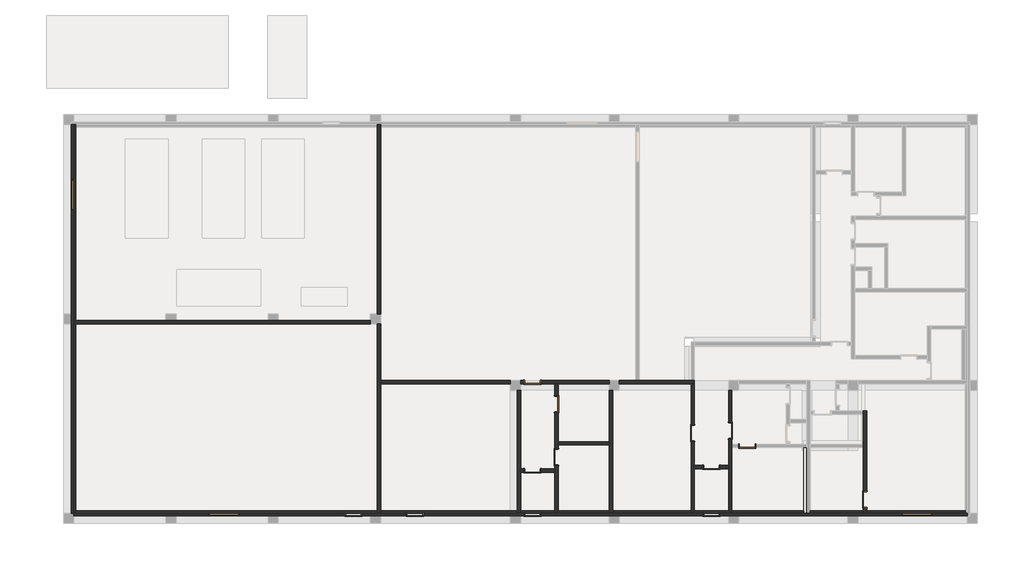
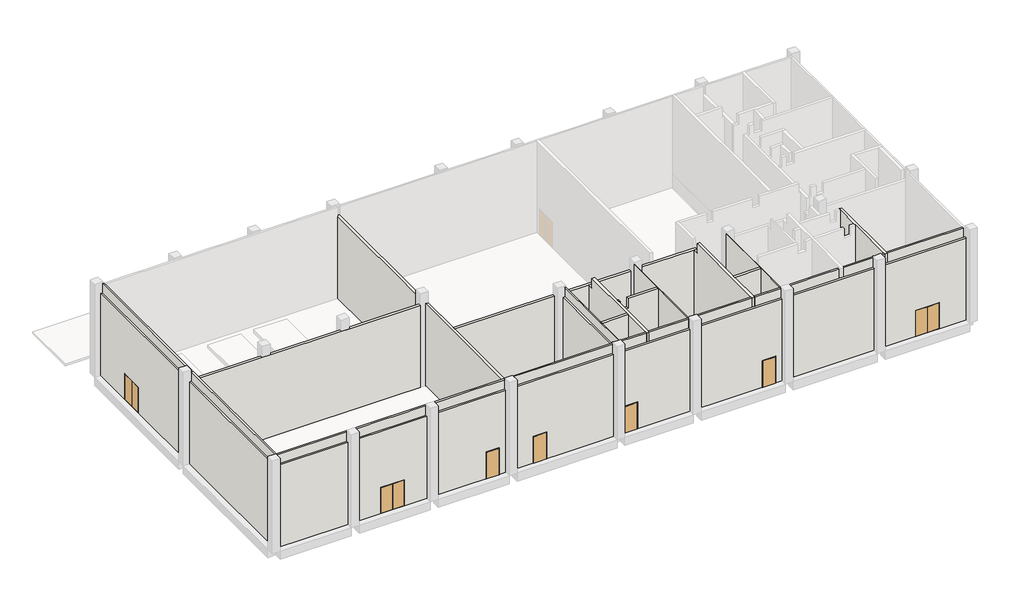
# One storey, part 1 of 4: 31 walls, 16 doors.
"""IFC4 building model written with IfcOpenShell, lengths in millimetres."""

import ifcopenshell
import ifcopenshell.guid

model = None  # the IFC model being written
_history = None  # IfcOwnerHistory: only IFC2X3 demands one
_inside = {}  # id of a spatial element -> (the spatial element, [elements in it])
_under = {}  # id of a project, library or spatial element -> (it, [spatial elements below it])
_declared = {}  # id of a project -> (the project, [libraries it declares])
_typed = {}  # id of a type object -> (the type object, [elements of that type])
_made_of = {}  # id of a material, layer set ... -> (it, [elements and type objects made of it])


def new_model(schema):
    """Start an empty IFC model of exactly this schema.

    Asked for "IFC4X3", IfcOpenShell would pick the latest addendum, in which some entities
    have other attributes; the version numbers below select the first issue.
    IFC2X3 requires an IfcOwnerHistory on every rooted entity: one is made here for all.
    """
    global model, _history
    if schema == "IFC4X3":
        model = ifcopenshell.file(schema_version=(4, 3, 0, 0))
    else:
        model = ifcopenshell.file(schema=schema)
    _inside.clear()
    _under.clear()
    _declared.clear()
    _typed.clear()
    _made_of.clear()
    _history = None
    if model.schema == "IFC2X3":
        org = make("IfcOrganization", Name="unknown")
        user = make(
            "IfcPersonAndOrganization",
            ThePerson=make("IfcPerson", FamilyName="unknown"),
            TheOrganization=org,
        )
        app = make(
            "IfcApplication",
            ApplicationDeveloper=org,
            Version="unknown",
            ApplicationFullName="unknown",
            ApplicationIdentifier="unknown",
        )
        _history = make(
            "IfcOwnerHistory",
            OwningUser=user,
            OwningApplication=app,
            ChangeAction="ADDED",
            CreationDate=0,
        )
    return model


def make(cls, **values):
    """One entity of the class cls with the attributes given. An attribute that is None is left unset."""
    return model.create_entity(
        cls, **{name: value for name, value in values.items() if value is not None}
    )


def rooted(cls, **values):
    """An entity with a GlobalId (a new one), such as an element, a storey or a relation."""
    return make(cls, GlobalId=ifcopenshell.guid.new(), OwnerHistory=_history, **values)


def si_unit(unit_type, name, prefix=None):
    """IfcSIUnit, for example si_unit("LENGTHUNIT", "METRE", prefix="MILLI")."""
    return make("IfcSIUnit", UnitType=unit_type, Prefix=prefix, Name=name)


def assignment(units):
    """IfcUnitAssignment: the units of a project."""
    return None if units is None else make("IfcUnitAssignment", Units=units)


def point(xyz):
    """IfcCartesianPoint."""
    return None if xyz is None else make("IfcCartesianPoint", Coordinates=xyz)


def direction(xyz):
    """IfcDirection."""
    return None if xyz is None else make("IfcDirection", DirectionRatios=xyz)


def frame(location, z_axis=None, x_axis=None):
    """IfcAxis2Placement3D, a coordinate frame: its origin and axes. An axis left out is left unset."""
    return make(
        "IfcAxis2Placement3D",
        Location=point(location),
        Axis=direction(z_axis),
        RefDirection=direction(x_axis),
    )


def origin():
    """The frame at (0, 0, 0) with its axes left unset."""
    return frame((0.0, 0.0, 0.0))


def origin_with_axes():
    """The frame at (0, 0, 0) with the z axis (0, 0, 1) and the x axis (1, 0, 0) written out."""
    return frame((0.0, 0.0, 0.0), z_axis=(0.0, 0.0, 1.0), x_axis=(1.0, 0.0, 0.0))


def place(relative_to, where):
    """IfcLocalPlacement: puts the frame where relative to a parent placement (None: the world)."""
    return make(
        "IfcLocalPlacement", PlacementRelTo=relative_to, RelativePlacement=where
    )


def context(
    kind, dimensions, precision=None, world=None, true_north=None, identifier=None
):
    """IfcGeometricRepresentationContext, for example the 3D "Model" context."""
    return make(
        "IfcGeometricRepresentationContext",
        ContextIdentifier=identifier,
        ContextType=kind,
        CoordinateSpaceDimension=dimensions,
        Precision=precision,
        WorldCoordinateSystem=world,
        TrueNorth=true_north,
    )


def project(units=None, contexts=None):
    """IfcProject with its units and contexts."""
    return rooted(
        "IfcProject",
        Name="project",
        RepresentationContexts=contexts,
        UnitsInContext=assignment(units),
    )


def spatial(cls, under=None, at=None, **own):
    """A site, building, storey or space (cls), placed at a placement, below another one or the project."""
    s = rooted(cls, ObjectPlacement=at, **own)
    if under is not None:
        _under.setdefault(under.id(), (under, []))[1].append(s)
    return s


def polyline(points):
    """IfcPolyline through the points."""
    return make("IfcPolyline", Points=[point(p) for p in points])


def outline(outer, holes=None, kind="AREA"):
    """IfcArbitraryClosedProfileDef: a profile drawn as a closed curve; with holes, ...WithVoids."""
    if holes is None:
        return make("IfcArbitraryClosedProfileDef", ProfileType=kind, OuterCurve=outer)
    return make(
        "IfcArbitraryProfileDefWithVoids",
        ProfileType=kind,
        OuterCurve=outer,
        InnerCurves=holes,
    )


def extrude(swept, where, along, depth):
    """IfcExtrudedAreaSolid: the profile swept, set in the frame where, extruded along a direction by depth."""
    return make(
        "IfcExtrudedAreaSolid",
        SweptArea=swept,
        Position=where,
        ExtrudedDirection=direction(along),
        Depth=depth,
    )


def faces_of(points, faces, orient=None, outer=None):
    """IfcFace entities. A face is a list of loops; a loop is a list of indices into points, from 0.

    orient and outer hold one flag for each loop. By default every Orientation is true, the
    first loop of a face is its IfcFaceOuterBound and the others are IfcFaceBound.
    """
    made = []
    for i, loops in enumerate(faces):
        bounds = []
        for j, loop in enumerate(loops):
            is_outer = j == 0 if outer is None else outer[i][j]
            bounds.append(
                make(
                    "IfcFaceOuterBound" if is_outer else "IfcFaceBound",
                    Bound=make("IfcPolyLoop", Polygon=[points[k] for k in loop]),
                    Orientation=True if orient is None else orient[i][j],
                )
            )
        made.append(make("IfcFace", Bounds=bounds))
    return made


def faceted_brep(points, faces, orient=None, outer=None, voids=None):
    """IfcFacetedBrep: a solid bounded by flat faces; with voids (closed shells), ...WithVoids."""
    shared = [point(p) for p in points]
    hull = make("IfcClosedShell", CfsFaces=faces_of(shared, faces, orient, outer))
    if voids is None:
        return make("IfcFacetedBrep", Outer=hull)
    return make(
        "IfcFacetedBrepWithVoids",
        Outer=hull,
        Voids=[
            make(cls, CfsFaces=faces_of(shared, fs, o, b)) for cls, fs, o, b in voids
        ],
    )


def shape(context_of_items, identifier, shape_type, items):
    """IfcShapeRepresentation: the items that make up one representation, for example the "Body"."""
    return make(
        "IfcShapeRepresentation",
        ContextOfItems=context_of_items,
        RepresentationIdentifier=identifier,
        RepresentationType=shape_type,
        Items=items,
    )


def source(mapping_origin, context_of_items, identifier, shape_type, items):
    """IfcRepresentationMap: a shape defined once, which mapped items show again and again."""
    return make(
        "IfcRepresentationMap",
        MappingOrigin=mapping_origin,
        MappedRepresentation=shape(context_of_items, identifier, shape_type, items),
    )


def transform(
    local_origin,
    x_axis=None,
    y_axis=None,
    z_axis=None,
    scale=None,
    scale2=None,
    scale3=None,
    uniform=True,
):
    """IfcCartesianTransformationOperator3D, or its non-uniform kind. x_axis, y_axis, z_axis: its Axis1, 2, 3."""
    if uniform:
        return make(
            "IfcCartesianTransformationOperator3D",
            Axis1=direction(x_axis),
            Axis2=direction(y_axis),
            LocalOrigin=point(local_origin),
            Scale=scale,
            Axis3=direction(z_axis),
        )
    return make(
        "IfcCartesianTransformationOperator3DnonUniform",
        Axis1=direction(x_axis),
        Axis2=direction(y_axis),
        LocalOrigin=point(local_origin),
        Scale=scale,
        Axis3=direction(z_axis),
        Scale2=scale2,
        Scale3=scale3,
    )


def mapped(mapping_source, mapping_target):
    """IfcMappedItem: shows the shape of a source again, moved by a transform."""
    return make(
        "IfcMappedItem", MappingSource=mapping_source, MappingTarget=mapping_target
    )


def made_of(thing, what):
    """Note that an element or type object is made of a material, layer set ...; save() writes the relation."""
    if what is not None:
        _made_of.setdefault(what.id(), (what, []))[1].append(thing)
    return thing


def element(
    cls,
    number,
    at=None,
    inside=None,
    cuts=None,
    type_object=None,
    material=None,
    context=None,
    identifier="Body",
    shape_type=None,
    held_by="IfcProductDefinitionShape",
    body=None,
    shapes=None,
    **own,
):
    """One element of the class cls, such as IfcWall. Its Tag is "e" and its number.

    at: its placement. inside: the storey or other place that contains it. cuts: it is an
    opening in that element (IfcRelVoidsElement). A single representation is given by context,
    identifier, shape_type and body (its items); several are given by shapes. held_by: the class
    of the entity that holds the representations. save() writes the other relations.
    """
    e = rooted(cls, Tag="e%d" % number, ObjectPlacement=at, **own)
    if body is not None:
        shapes = [shape(context, identifier, shape_type, body)]
    if shapes is not None:
        e.Representation = make(held_by, Representations=shapes)
    if inside is not None:
        _inside.setdefault(inside.id(), (inside, []))[1].append(e)
    if cuts is not None:
        rooted(
            "IfcRelVoidsElement", RelatingBuildingElement=cuts, RelatedOpeningElement=e
        )
    if type_object is not None:
        _typed.setdefault(type_object.id(), (type_object, []))[1].append(e)
    return made_of(e, material)


def aggregate(whole, parts):
    """IfcRelAggregates: a whole, such as a stair, and the parts it consists of."""
    return rooted("IfcRelAggregates", RelatingObject=whole, RelatedObjects=parts)


def save(model, path):
    """Write the relations noted so far, then the file.

    IfcRelAggregates (storeys below a building ...), IfcRelContainedInSpatialStructure (elements
    in a storey), IfcRelDefinesByType, IfcRelAssociatesMaterial and IfcRelDeclares: one each for
    every whole, place, type object, material and project.
    """
    for whole, parts in _under.values():
        aggregate(whole, parts)
    for where, things in _inside.values():
        rooted(
            "IfcRelContainedInSpatialStructure",
            RelatedElements=things,
            RelatingStructure=where,
        )
    for kind, things in _typed.values():
        rooted("IfcRelDefinesByType", RelatedObjects=things, RelatingType=kind)
    for what, things in _made_of.values():
        rooted("IfcRelAssociatesMaterial", RelatedObjects=things, RelatingMaterial=what)
    for by, libraries in _declared.values():
        rooted("IfcRelDeclares", RelatingContext=by, RelatedDefinitions=libraries)
    model.write(path)


def double_door_steel_580823b0(model_context):
    return source(origin(), model_context, "Body", "SolidModel", [
        extrude(outline(polyline([(880.0, 35.0), (0.0, 35.0), (0.0, 75.0), (880.0, 75.0), (880.0, 35.0)])), frame((0.0, 0.0, 20.0), z_axis=(0.0, 0.0, 1.0), x_axis=(1.0, 0.0, 0.0)), (0.0, 0.0, 1.0), 2060.0),
        extrude(outline(polyline([(0.0, 35.0), (-880.0, 35.0), (-880.0, 75.0), (0.0, 75.0), (0.0, 35.0)])), frame((0.0, 0.0, 20.0), z_axis=(0.0, 0.0, 1.0), x_axis=(1.0, 0.0, 0.0)), (0.0, 0.0, 1.0), 2060.0),
        faceted_brep([(900.0, -75.0, 2100.0), (900.0, 75.0, 2100.0), (-900.0, 75.0, 2100.0), (-900.0, -75.0, 2100.0), (865.0, 35.0, 2065.0), (865.0, -75.0, 2065.0), (-865.0, -75.0, 2065.0), (-865.0, 35.0, 2065.0), (880.0, 75.0, 2080.0), (880.0, 35.0, 2080.0), (-880.0, 35.0, 2080.0), (-880.0, 75.0, 2080.0), (-900.0, 75.0, 0.0), (-900.0, -75.0, 0.0), (-865.0, -75.0, 35.0), (-865.0, 35.0, 35.0), (-880.0, 35.0, 20.0), (-880.0, 75.0, 20.0), (900.0, 75.0, 0.0), (880.0, 75.0, 20.0), (900.0, -75.0, 0.0), (865.0, -75.0, 35.0), (865.0, 35.0, 35.0), (880.0, 35.0, 20.0)], [[[0, 1, 2, 3]], [[4, 5, 6, 7]], [[8, 9, 10, 11]], [[3, 2, 12, 13]], [[7, 6, 14, 15]], [[11, 10, 16, 17]], [[18, 12, 2, 1], [8, 11, 17, 19]], [[13, 12, 18, 20]], [[0, 3, 13, 20], [21, 14, 6, 5]], [[15, 14, 21, 22]], [[23, 16, 10, 9], [4, 7, 15, 22]], [[17, 16, 23, 19]], [[20, 18, 1, 0]], [[22, 21, 5, 4]], [[19, 23, 9, 8]]]),
    ])


def single_door_steel_b319cbd1(model_context):
    return source(origin(), model_context, "Body", "SolidModel", [
        extrude(outline(polyline([(480.0, -105.0), (-480.0, -105.0), (-480.0, -70.0), (480.0, -70.0), (480.0, -105.0)])), origin_with_axes(), (0.0, 0.0, 1.0), 2130.0),
        faceted_brep([(480.0, -105.0, 0.0), (480.0, -70.0, 0.0), (460.0, -70.0, 0.0), (460.0, 70.0, 0.0), (480.0, 70.0, 0.0), (480.0, 105.0, 0.0), (510.0, 105.0, 0.0), (510.0, -105.0, 0.0), (510.0, -105.0, 2160.0), (-510.0, -105.0, 2160.0), (-510.0, -105.0, 0.0), (-480.0, -105.0, 0.0), (-480.0, -105.0, 2130.0), (480.0, -105.0, 2130.0), (510.0, 105.0, 2160.0), (480.0, 105.0, 2130.0), (-480.0, 105.0, 2130.0), (-480.0, 105.0, 0.0), (-510.0, 105.0, 0.0), (-510.0, 105.0, 2160.0), (480.0, 70.0, 2130.0), (460.0, 70.0, 2110.0), (-460.0, 70.0, 2110.0), (-460.0, 70.0, 0.0), (-480.0, 70.0, 0.0), (-480.0, 70.0, 2130.0), (460.0, -70.0, 2110.0), (480.0, -70.0, 2130.0), (-480.0, -70.0, 2130.0), (-480.0, -70.0, 0.0), (-460.0, -70.0, 0.0), (-460.0, -70.0, 2110.0)], [[[0, 1, 2, 3, 4, 5, 6, 7]], [[7, 8, 9, 10, 11, 12, 13, 0]], [[6, 14, 8, 7]], [[5, 15, 16, 17, 18, 19, 14, 6]], [[4, 20, 15, 5]], [[3, 21, 22, 23, 24, 25, 20, 4]], [[2, 26, 21, 3]], [[1, 27, 28, 29, 30, 31, 26, 2]], [[0, 13, 27, 1]], [[12, 11, 29, 28]], [[11, 10, 18, 17, 24, 23, 30, 29]], [[19, 18, 10, 9]], [[25, 24, 17, 16]], [[31, 30, 23, 22]], [[14, 19, 9, 8]], [[20, 25, 16, 15]], [[26, 31, 22, 21]], [[13, 12, 28, 27]]]),
    ])


def single_door_steel_f73fbc53(model_context):
    return source(origin(), model_context, "Body", "SolidModel", [
        extrude(outline(polyline([(480.0, -130.0), (-480.0, -130.0), (-480.0, -95.0), (480.0, -95.0), (480.0, -130.0)])), origin_with_axes(), (0.0, 0.0, 1.0), 2130.0),
        faceted_brep([(480.0, -130.0, 0.0), (480.0, -95.0, 0.0), (460.0, -95.0, 0.0), (460.0, 95.0, 0.0), (480.0, 95.0, 0.0), (480.0, 130.0, 0.0), (510.0, 130.0, 0.0), (510.0, -130.0, 0.0), (510.0, -130.0, 2160.0), (-510.0, -130.0, 2160.0), (-510.0, -130.0, 0.0), (-480.0, -130.0, 0.0), (-480.0, -130.0, 2130.0), (480.0, -130.0, 2130.0), (510.0, 130.0, 2160.0), (480.0, 130.0, 2130.0), (-480.0, 130.0, 2130.0), (-480.0, 130.0, 0.0), (-510.0, 130.0, 0.0), (-510.0, 130.0, 2160.0), (480.0, 95.0, 2130.0), (460.0, 95.0, 2110.0), (-460.0, 95.0, 2110.0), (-460.0, 95.0, 0.0), (-480.0, 95.0, 0.0), (-480.0, 95.0, 2130.0), (460.0, -95.0, 2110.0), (480.0, -95.0, 2130.0), (-480.0, -95.0, 2130.0), (-480.0, -95.0, 0.0), (-460.0, -95.0, 0.0), (-460.0, -95.0, 2110.0)], [[[0, 1, 2, 3, 4, 5, 6, 7]], [[7, 8, 9, 10, 11, 12, 13, 0]], [[6, 14, 8, 7]], [[5, 15, 16, 17, 18, 19, 14, 6]], [[4, 20, 15, 5]], [[3, 21, 22, 23, 24, 25, 20, 4]], [[2, 26, 21, 3]], [[1, 27, 28, 29, 30, 31, 26, 2]], [[0, 13, 27, 1]], [[12, 11, 29, 28]], [[11, 10, 18, 17, 24, 23, 30, 29]], [[19, 18, 10, 9]], [[25, 24, 17, 16]], [[31, 30, 23, 22]], [[14, 19, 9, 8]], [[20, 25, 16, 15]], [[26, 31, 22, 21]], [[13, 12, 28, 27]]]),
    ])


def single_door_steel_4bf023c6(model_context):
    return source(origin(), model_context, "Body", "SolidModel", [
        extrude(outline(polyline([(480.0, 130.0), (480.0, 95.0), (-480.0, 95.0), (-480.0, 130.0), (480.0, 130.0)])), origin_with_axes(), (0.0, 0.0, 1.0), 2130.0),
        faceted_brep([(480.0, 130.0, 0.0), (510.0, 130.0, 0.0), (510.0, -130.0, 0.0), (480.0, -130.0, 0.0), (480.0, -95.0, 0.0), (460.0, -95.0, 0.0), (460.0, 95.0, 0.0), (480.0, 95.0, 0.0), (480.0, 130.0, 2130.0), (-480.0, 130.0, 2130.0), (-480.0, 130.0, 0.0), (-510.0, 130.0, 0.0), (-510.0, 130.0, 2160.0), (510.0, 130.0, 2160.0), (510.0, -130.0, 2160.0), (-510.0, -130.0, 2160.0), (-510.0, -130.0, 0.0), (-480.0, -130.0, 0.0), (-480.0, -130.0, 2130.0), (480.0, -130.0, 2130.0), (480.0, -95.0, 2130.0), (-480.0, -95.0, 2130.0), (-480.0, -95.0, 0.0), (-460.0, -95.0, 0.0), (-460.0, -95.0, 2110.0), (460.0, -95.0, 2110.0), (460.0, 95.0, 2110.0), (-460.0, 95.0, 2110.0), (-460.0, 95.0, 0.0), (-480.0, 95.0, 0.0), (-480.0, 95.0, 2130.0), (480.0, 95.0, 2130.0)], [[[0, 1, 2, 3, 4, 5, 6, 7]], [[1, 0, 8, 9, 10, 11, 12, 13]], [[2, 1, 13, 14]], [[3, 2, 14, 15, 16, 17, 18, 19]], [[4, 3, 19, 20]], [[5, 4, 20, 21, 22, 23, 24, 25]], [[6, 5, 25, 26]], [[7, 6, 26, 27, 28, 29, 30, 31]], [[0, 7, 31, 8]], [[9, 30, 29, 10]], [[10, 29, 28, 23, 22, 17, 16, 11]], [[15, 12, 11, 16]], [[21, 18, 17, 22]], [[27, 24, 23, 28]], [[14, 13, 12, 15]], [[20, 19, 18, 21]], [[26, 25, 24, 27]], [[8, 31, 30, 9]]]),
    ])


def single_door_steel_ed84bdaa(model_context):
    return source(origin(), model_context, "Body", "SolidModel", [
        extrude(outline(polyline([(480.0, 105.0), (480.0, 70.0), (-480.0, 70.0), (-480.0, 105.0), (480.0, 105.0)])), origin_with_axes(), (0.0, 0.0, 1.0), 2130.0),
        faceted_brep([(480.0, 105.0, 0.0), (510.0, 105.0, 0.0), (510.0, -105.0, 0.0), (480.0, -105.0, 0.0), (480.0, -70.0, 0.0), (460.0, -70.0, 0.0), (460.0, 70.0, 0.0), (480.0, 70.0, 0.0), (480.0, 105.0, 2130.0), (-480.0, 105.0, 2130.0), (-480.0, 105.0, 0.0), (-510.0, 105.0, 0.0), (-510.0, 105.0, 2160.0), (510.0, 105.0, 2160.0), (510.0, -105.0, 2160.0), (-510.0, -105.0, 2160.0), (-510.0, -105.0, 0.0), (-480.0, -105.0, 0.0), (-480.0, -105.0, 2130.0), (480.0, -105.0, 2130.0), (480.0, -70.0, 2130.0), (-480.0, -70.0, 2130.0), (-480.0, -70.0, 0.0), (-460.0, -70.0, 0.0), (-460.0, -70.0, 2110.0), (460.0, -70.0, 2110.0), (460.0, 70.0, 2110.0), (-460.0, 70.0, 2110.0), (-460.0, 70.0, 0.0), (-480.0, 70.0, 0.0), (-480.0, 70.0, 2130.0), (480.0, 70.0, 2130.0)], [[[0, 1, 2, 3, 4, 5, 6, 7]], [[1, 0, 8, 9, 10, 11, 12, 13]], [[2, 1, 13, 14]], [[3, 2, 14, 15, 16, 17, 18, 19]], [[4, 3, 19, 20]], [[5, 4, 20, 21, 22, 23, 24, 25]], [[6, 5, 25, 26]], [[7, 6, 26, 27, 28, 29, 30, 31]], [[0, 7, 31, 8]], [[9, 30, 29, 10]], [[10, 29, 28, 23, 22, 17, 16, 11]], [[15, 12, 11, 16]], [[21, 18, 17, 22]], [[27, 24, 23, 28]], [[14, 13, 12, 15]], [[20, 19, 18, 21]], [[26, 25, 24, 27]], [[8, 31, 30, 9]]]),
    ])


model = new_model("IFC4")

# Units and contexts
model_context = context("Model", 3, world=origin())
ifc_project = project(units=[si_unit("LENGTHUNIT", "METRE", prefix="MILLI")], contexts=[model_context])

# Site, building, storey
site = spatial("IfcSite", under=ifc_project)
building = spatial("IfcBuilding", under=site)
storey = spatial("IfcBuildingStorey", under=building, Name="TOC(GF)", Elevation=97049.9618634)

# Doors
placement = place(None, origin())
double_door_steel_shape = double_door_steel_580823b0(model_context)
element("IfcDoor", 1, ObjectType="Double Door_Steel : H_DR_AR B12_Door_Double SD 02", at=placement, inside=storey, context=model_context, shape_type="MappedRepresentation", body=[
    mapped(double_door_steel_shape, transform((49750.0, -19275.0, 97049.9618634), x_axis=(-1.0, 0.0, 0.0), y_axis=(0.0, -1.0, 0.0), z_axis=(0.0, 0.0, 1.0))),
])
element("IfcDoor", 2, ObjectType="Double Door_Steel : H_DR_AR B12_Door_Double FSD 02", at=placement, inside=storey, context=model_context, shape_type="MappedRepresentation", body=[
    mapped(double_door_steel_shape, transform((9100.0, -19275.0, 97049.9618634), x_axis=(-1.0, 0.0, 0.0), y_axis=(0.0, -1.0, 0.0), z_axis=(0.0, 0.0, 1.0))),
])
element("IfcDoor", 3, ObjectType="Double Door_Steel : H_DR_AR B12_Door_Double FSD 02", at=placement, inside=storey, context=model_context, shape_type="MappedRepresentation", body=[
    mapped(double_door_steel_shape, transform((225.0, -500.0, 97049.9618634), x_axis=(0.0, 1.0, 0.0), y_axis=(-1.0, 0.0, 0.0), z_axis=(0.0, 0.0, 1.0))),
])
single_door_steel_shape = single_door_steel_b319cbd1(model_context)
element("IfcDoor", 4, ObjectType="Single Door_Steel : H_DR_AR B12_Door_Single FSD 01", at=placement, inside=storey, context=model_context, shape_type="MappedRepresentation", body=[
    mapped(single_door_steel_shape, transform((27200.0, -19275.0, 97049.9618634), x_axis=(1.0, 0.0, 0.0), y_axis=(0.0, 1.0, 0.0), z_axis=(0.0, 0.0, 1.0))),
])
element("IfcDoor", 5, ObjectType="Single Door_Steel : H_DR_AR B12_Door_Single FSD 01", at=placement, inside=storey, context=model_context, shape_type="MappedRepresentation", body=[
    mapped(single_door_steel_shape, transform((20300.0, -19275.0, 97049.9618634), x_axis=(1.0, 0.0, 0.0), y_axis=(0.0, 1.0, 0.0), z_axis=(0.0, 0.0, 1.0))),
])
single_door_steel_2_shape = single_door_steel_f73fbc53(model_context)
element("IfcDoor", 6, ObjectType="Single Door_Steel : H_DR_AR B12_Door_Single FSD 01", at=placement, inside=storey, context=model_context, shape_type="MappedRepresentation", body=[
    mapped(single_door_steel_2_shape, transform((28600.0, -15900.0, 97049.9618634), x_axis=(0.0, -1.0, 0.0), y_axis=(1.0, 0.0, 0.0), z_axis=(0.0, 0.0, 1.0))),
])
element("IfcDoor", 7, ObjectType="Single Door_Steel : H_DR_AR B12_Door_Single FSD 01", at=placement, inside=storey, context=model_context, shape_type="MappedRepresentation", body=[
    mapped(single_door_steel_2_shape, transform((27200.0, -16700.0, 97049.9618634), x_axis=(1.0, 0.0, 0.0), y_axis=(0.0, 1.0, 0.0), z_axis=(0.0, 0.0, 1.0))),
])
element("IfcDoor", 8, ObjectType="Single Door_Steel : H_DR_AR B12_Door_Single FSD 01", at=placement, inside=storey, context=model_context, shape_type="MappedRepresentation", body=[
    mapped(single_door_steel_2_shape, transform((27200.0, -11500.0, 97049.9618634), x_axis=(1.0, 0.0, 0.0), y_axis=(0.0, 1.0, 0.0), z_axis=(0.0, 0.0, 1.0))),
])
single_door_steel_3_shape = single_door_steel_4bf023c6(model_context)
element("IfcDoor", 9, ObjectType="Single Door_Steel : H_DR_AR B12_Door_Single FSD 01", at=placement, inside=storey, context=model_context, shape_type="MappedRepresentation", body=[
    mapped(single_door_steel_3_shape, transform((39800.0, -15250.0, 97049.9618634), x_axis=(-1.0, 0.0, 0.0), y_axis=(0.0, -1.0, 0.0), z_axis=(0.0, 0.0, 1.0))),
])
element("IfcDoor", 10, ObjectType="Single Door_Steel : H_DR_AR B12_Door_Single FSD 01", at=placement, inside=storey, context=model_context, shape_type="MappedRepresentation", body=[
    mapped(single_door_steel_3_shape, transform((38800.0, -14350.0, 97049.9618634), x_axis=(0.0, -1.0, 0.0), y_axis=(1.0, 0.0, 0.0), z_axis=(0.0, 0.0, 1.0))),
])
element("IfcDoor", 11, ObjectType="Single Door_Steel : H_DR_AR B12_Door_Single FSD 01", at=placement, inside=storey, context=model_context, shape_type="MappedRepresentation", body=[
    mapped(single_door_steel_3_shape, transform((46700.0, -18400.0, 97049.9618634), x_axis=(0.0, 1.0, 0.0), y_axis=(-1.0, 0.0, 0.0), z_axis=(0.0, 0.0, 1.0))),
])
element("IfcDoor", 12, ObjectType="Single Door_Steel : H_DR_AR B12_Door_Single FSD 01", at=placement, inside=storey, context=model_context, shape_type="MappedRepresentation", body=[
    mapped(single_door_steel_3_shape, transform((36600.0, -14500.0, 97049.9618634), x_axis=(0.0, 1.0, 0.0), y_axis=(-1.0, 0.0, 0.0), z_axis=(0.0, 0.0, 1.0))),
])
element("IfcDoor", 13, ObjectType="Single Door_Steel : H_DR_AR B12_Door_Single FSD 01", at=placement, inside=storey, context=model_context, shape_type="MappedRepresentation", body=[
    mapped(single_door_steel_3_shape, transform((37700.0, -16500.0, 97049.9618634), x_axis=(-1.0, 0.0, 0.0), y_axis=(0.0, -1.0, 0.0), z_axis=(0.0, 0.0, 1.0))),
])
element("IfcDoor", 14, ObjectType="Single Door_Steel : H_DR_AR B12_Door_Single FSD 01", at=placement, inside=storey, context=model_context, shape_type="MappedRepresentation", body=[
    mapped(single_door_steel_3_shape, transform((28600.0, -12800.0, 97049.9618634), x_axis=(0.0, -1.0, 0.0), y_axis=(1.0, 0.0, 0.0), z_axis=(0.0, 0.0, 1.0))),
])
single_door_steel_4_shape = single_door_steel_ed84bdaa(model_context)
element("IfcDoor", 15, ObjectType="Single Door_Steel : H_DR_AR B12_Door_Single FSD 01", at=placement, inside=storey, context=model_context, shape_type="MappedRepresentation", body=[
    mapped(single_door_steel_4_shape, transform((37700.0, -19275.0, 97049.9618634), x_axis=(-1.0, 0.0, 0.0), y_axis=(0.0, -1.0, 0.0), z_axis=(0.0, 0.0, 1.0))),
])
element("IfcDoor", 16, ObjectType="Single Door_Steel : H_DR_AR B12_Door_Single FSD 01", at=placement, inside=storey, context=model_context, shape_type="MappedRepresentation", body=[
    mapped(single_door_steel_4_shape, transform((16700.0, -19275.0, 97049.9618634), x_axis=(-1.0, 0.0, 0.0), y_axis=(0.0, -1.0, 0.0), z_axis=(0.0, 0.0, 1.0))),
])

# Walls
element("IfcWall", 17, ObjectType="H_WA_AR B02_Ext Wall RC-AG_EW5", at=placement, inside=storey, context=model_context, shape_type="Brep", body=[
    faceted_brep([(52700.0, -19200.0, 97049.9618634), (52574.0, -19200.0, 97049.9618634), (50650.0, -19200.0, 97049.9618634), (50650.0, -19200.0, 99149.9618634), (48850.0, -19200.0, 99149.9618634), (48850.0, -19200.0, 97049.9618634), (46800.0, -19200.0, 97049.9618634), (46600.0, -19200.0, 97049.9618634), (43500.0, -19200.0, 97049.9618634), (43300.0, -19200.0, 97049.9618634), (43100.0, -19200.0, 97049.9618634), (38900.0, -19200.0, 97049.9618634), (38700.0, -19200.0, 97049.9618634), (38210.0, -19200.0, 97049.9618634), (38210.0, -19200.0, 99209.9618634), (37190.0, -19200.0, 99209.9618634), (37190.0, -19200.0, 97049.9618634), (36700.0, -19200.0, 97049.9618634), (36500.0, -19200.0, 97049.9618634), (31900.0, -19200.0, 97049.9618634), (31700.0, -19200.0, 97049.9618634), (28700.0, -19200.0, 97049.9618634), (28500.0, -19200.0, 97049.9618634), (27710.0, -19200.0, 97049.9618634), (27710.0, -19200.0, 99209.9618634), (26690.0, -19200.0, 99209.9618634), (26690.0, -19200.0, 97049.9618634), (26500.0, -19200.0, 97049.9618634), (26300.0, -19200.0, 97049.9618634), (20810.0, -19200.0, 97049.9618634), (20810.0, -19200.0, 99209.9618634), (19790.0, -19200.0, 99209.9618634), (19790.0, -19200.0, 97049.9618634), (18300.0, -19200.0, 97049.9618634), (18100.0, -19200.0, 97049.9618634), (17210.0, -19200.0, 97049.9618634), (17210.0, -19200.0, 99209.9618634), (16190.0, -19200.0, 99209.9618634), (16190.0, -19200.0, 97049.9618634), (10000.0, -19200.0, 97049.9618634), (10000.0, -19200.0, 99149.9618634), (8200.0, -19200.0, 99149.9618634), (8200.0, -19200.0, 97049.9618634), (426.0, -19200.0, 97049.9618634), (300.0, -19200.0, 97049.9618634), (300.0, -19200.0, 103650.0), (5700.0, -19200.0, 103650.0), (6300.0, -19200.0, 103650.0), (11700.0, -19200.0, 103650.0), (12300.0, -19200.0, 103650.0), (17700.0, -19200.0, 103650.0), (18100.0, -19200.0, 103650.0), (18300.0, -19200.0, 103650.0), (25900.0, -19200.0, 103650.0), (26300.0, -19200.0, 103650.0), (26450.0, -19200.0, 103650.0), (26500.0, -19200.0, 103650.0), (31700.0, -19200.0, 103650.0), (31750.0, -19200.0, 103650.0), (31900.0, -19200.0, 103650.0), (32300.0, -19200.0, 103650.0), (38700.0, -19200.0, 103650.0), (38750.0, -19200.0, 103650.0), (38900.0, -19200.0, 103650.0), (39300.0, -19200.0, 103650.0), (45700.0, -19200.0, 103650.0), (46300.0, -19200.0, 103650.0), (52700.0, -19200.0, 103650.0), (50650.0, -19350.0, 97049.9618634), (52700.0, -19350.0, 97049.9618634), (52700.0, -19350.0, 103650.0), (300.0, -19350.0, 103650.0), (300.0, -19350.0, 97049.9618634), (8200.0, -19350.0, 97049.9618634), (8200.0, -19350.0, 99149.9618634), (10000.0, -19350.0, 99149.9618634), (10000.0, -19350.0, 97049.9618634), (16190.0, -19350.0, 97049.9618634), (16190.0, -19350.0, 99209.9618634), (17210.0, -19350.0, 99209.9618634), (17210.0, -19350.0, 97049.9618634), (19790.0, -19350.0, 97049.9618634), (19790.0, -19350.0, 99209.9618634), (20810.0, -19350.0, 99209.9618634), (20810.0, -19350.0, 97049.9618634), (26690.0, -19350.0, 97049.9618634), (26690.0, -19350.0, 99209.9618634), (27710.0, -19350.0, 99209.9618634), (27710.0, -19350.0, 97049.9618634), (37190.0, -19350.0, 97049.9618634), (37190.0, -19350.0, 99209.9618634), (38210.0, -19350.0, 99209.9618634), (38210.0, -19350.0, 97049.9618634), (48850.0, -19350.0, 97049.9618634), (48850.0, -19350.0, 99149.9618634), (50650.0, -19350.0, 99149.9618634)], [[[0, 1, 2, 3, 4, 5, 6, 7, 8, 9, 10, 11, 12, 13, 14, 15, 16, 17, 18, 19, 20, 21, 22, 23, 24, 25, 26, 27, 28, 29, 30, 31, 32, 33, 34, 35, 36, 37, 38, 39, 40, 41, 42, 43, 44, 45, 46, 47, 48, 49, 50, 51, 52, 53, 54, 55, 56, 57, 58, 59, 60, 61, 62, 63, 64, 65, 66, 67]], [[68, 69, 70, 71, 72, 73, 74, 75, 76, 77, 78, 79, 80, 81, 82, 83, 84, 85, 86, 87, 88, 89, 90, 91, 92, 93, 94, 95]], [[0, 69, 68, 2, 1]], [[5, 93, 92, 13, 12, 11, 10, 9, 8, 7, 6]], [[16, 89, 88, 23, 22, 21, 20, 19, 18, 17]], [[26, 85, 84, 29, 28, 27]], [[32, 81, 80, 35, 34, 33]], [[38, 77, 76, 39]], [[42, 73, 72, 44, 43]], [[69, 0, 67, 70]], [[70, 67, 66, 65, 64, 63, 62, 61, 60, 59, 58, 57, 56, 55, 54, 53, 52, 51, 50, 49, 48, 47, 46, 45, 71]], [[4, 94, 93, 5]], [[94, 4, 3, 95]], [[95, 3, 2, 68]], [[15, 90, 89, 16]], [[90, 15, 14, 91]], [[91, 14, 13, 92]], [[24, 23, 88, 87]], [[25, 24, 87, 86]], [[26, 25, 86, 85]], [[30, 29, 84, 83]], [[31, 30, 83, 82]], [[32, 31, 82, 81]], [[37, 78, 77, 38]], [[78, 37, 36, 79]], [[79, 36, 35, 80]], [[41, 74, 73, 42]], [[74, 41, 40, 75]], [[75, 40, 39, 76]], [[45, 44, 72, 71]]]),
])
element("IfcWall", 18, ObjectType="H_WA_AR B02_Ext Wall RC-AG_EW5", at=placement, inside=storey, context=model_context, shape_type="Brep", body=[
    faceted_brep([(300.0, 3600.0, 103650.0), (300.0, -7500.0, 103650.0), (300.0, -7900.0, 103650.0), (300.0, -8100.0, 103650.0), (300.0, -19200.0, 103650.0), (300.0, -19200.0, 97049.9618634), (300.0, -8100.0, 97049.9618634), (300.0, -7900.0, 97049.9618634), (300.0, -1400.0, 97049.9618634), (300.0, -1400.0, 99149.9618634), (300.0, 400.0, 99149.9618634), (300.0, 400.0, 97049.9618634), (300.0, 3600.0, 97049.9618634), (150.0, -19200.0, 97049.9618634), (150.0, -19200.0, 103650.0), (150.0, 3600.0, 103650.0), (150.0, 3600.0, 97049.9618634), (150.0, 400.0, 97049.9618634), (150.0, 400.0, 99149.9618634), (150.0, -1400.0, 99149.9618634), (150.0, -1400.0, 97049.9618634)], [[[0, 1, 2, 3, 4, 5, 6, 7, 8, 9, 10, 11, 12]], [[13, 14, 15, 16, 17, 18, 19, 20]], [[5, 13, 20, 8, 7, 6]], [[16, 12, 11, 17]], [[12, 16, 15, 0]], [[13, 5, 4, 14]], [[0, 15, 14, 4, 3, 2, 1]], [[10, 18, 17, 11]], [[18, 10, 9, 19]], [[19, 9, 8, 20]]]),
])
element("IfcWall", 19, ObjectType="H_WA_AR_B02_Ext Wall_RC_T200_W2", at=placement, inside=storey, context=model_context, shape_type="Brep", body=[
    faceted_brep([(36400.0, -11400.0, 98049.9618634), (36400.0, -11400.0, 97049.9618634), (33450.0, -11400.0, 97049.9618634), (33250.0, -11400.0, 97049.9618634), (27710.0, -11400.0, 97049.9618634), (27710.0, -11400.0, 98049.9618634), (31700.0, -11400.0, 98049.9618634), (32300.0, -11400.0, 98049.9618634), (36400.0, -11600.0, 97049.9618634), (36400.0, -11600.0, 98049.9618634), (32300.0, -11600.0, 98049.9618634), (31700.0, -11600.0, 98049.9618634), (27710.0, -11600.0, 98049.9618634), (27710.0, -11600.0, 97049.9618634), (28500.0, -11600.0, 97049.9618634), (28700.0, -11600.0, 97049.9618634)], [[[0, 1, 2, 3, 4, 5, 6, 7]], [[8, 9, 10, 11, 12, 13, 14, 15]], [[1, 8, 15, 14, 13, 4, 3, 2]], [[9, 0, 7, 6, 5, 12, 11, 10]], [[1, 0, 9, 8]], [[5, 4, 13, 12]]]),
    faceted_brep([(26690.0, -11400.0, 98049.9618634), (26690.0, -11400.0, 97049.9618634), (26500.0, -11400.0, 97049.9618634), (26500.0, -11400.0, 98049.9618634), (26690.0, -11600.0, 97049.9618634), (26690.0, -11600.0, 98049.9618634), (26500.0, -11600.0, 98049.9618634), (26500.0, -11600.0, 97049.9618634)], [[[0, 1, 2, 3]], [[4, 5, 6, 7]], [[1, 4, 7, 2]], [[5, 0, 3, 6]], [[1, 0, 5, 4]], [[3, 2, 7, 6]]]),
])
element("IfcWall", 20, ObjectType="H_WA_AR_B02_Ext Wall_RC_T200_W2", at=placement, inside=storey, context=model_context, shape_type="Brep", body=[
    faceted_brep([(26300.0, -19200.0, 97049.9618634), (26300.0, -19200.0, 98049.9618634), (26300.0, -19074.0, 98049.9618634), (26300.0, -12000.0, 98049.9618634), (26300.0, -12000.0, 97049.9618634), (26300.0, -19074.0, 97049.9618634), (26500.0, -19200.0, 98049.9618634), (26500.0, -19200.0, 97049.9618634), (26500.0, -19074.0, 97049.9618634), (26500.0, -16800.0, 97049.9618634), (26500.0, -16600.0, 97049.9618634), (26500.0, -12000.0, 97049.9618634), (26500.0, -12000.0, 98049.9618634), (26500.0, -19074.0, 98049.9618634)], [[[0, 1, 2, 3, 4, 5]], [[6, 7, 8, 9, 10, 11, 12, 13]], [[7, 0, 5, 4, 11, 10, 9, 8]], [[1, 6, 13, 12, 3, 2]], [[1, 0, 7, 6]], [[4, 3, 12, 11]]]),
])
element("IfcWall", 21, ObjectType="H_WA_AR_B02_Ext Wall_RC_T200_W2", at=placement, inside=storey, context=model_context, shape_type="Brep", body=[
    faceted_brep([(43100.0, -15150.0, 97049.9618634), (43100.0, -15350.0, 97049.9618634), (43100.0, -19074.0, 97049.9618634), (43100.0, -19200.0, 97049.9618634), (43100.0, -19200.0, 98049.9618634), (43100.0, -15350.0, 98049.9618634), (43100.0, -15150.0, 98049.9618634), (43300.0, -15150.0, 97049.9618634), (43300.0, -15150.0, 98049.9618634), (43300.0, -15350.0, 98049.9618634), (43300.0, -19200.0, 98049.9618634), (43300.0, -19200.0, 97049.9618634)], [[[0, 1, 2, 3, 4, 5, 6]], [[7, 8, 9, 10, 11]], [[3, 2, 1, 0, 7, 11]], [[6, 5, 4, 10, 9, 8]], [[0, 6, 8, 7]], [[4, 3, 11, 10]]]),
])
element("IfcWall", 22, ObjectType="H_WA_AR B02_Int Wall MA_IW1 T200", at=placement, inside=storey, context=model_context, shape_type="Brep", body=[
    faceted_brep([(300.0, -8100.0, 97049.9618634), (426.0, -8100.0, 97049.9618634), (17700.0, -8100.0, 97049.9618634), (17700.0, -8100.0, 103650.0), (12300.0, -8100.0, 103650.0), (11700.0, -8100.0, 103650.0), (6300.0, -8100.0, 103650.0), (5700.0, -8100.0, 103650.0), (300.0, -8100.0, 103650.0), (17700.0, -7900.0, 97049.9618634), (426.0, -7900.0, 97049.9618634), (300.0, -7900.0, 97049.9618634), (300.0, -7900.0, 103650.0), (17700.0, -7900.0, 103650.0)], [[[0, 1, 2, 3, 4, 5, 6, 7, 8]], [[9, 10, 11, 12, 13]], [[2, 1, 0, 11, 10, 9]], [[2, 9, 13, 3]], [[11, 0, 8, 12]], [[12, 8, 7, 6, 5, 4, 3, 13]]]),
])
element("IfcWall", 23, ObjectType="H_WA_AR B02_Int Wall MA_IW1 T200", at=placement, inside=storey, context=model_context, shape_type="Brep", body=[
    faceted_brep([(18300.0, -7500.0, 97049.9618634), (18300.0, 3474.0, 97049.9618634), (18300.0, 3600.0, 97049.9618634), (18300.0, 3600.0, 103650.0), (18300.0, -7500.0, 103650.0), (18100.0, 3600.0, 97049.9618634), (18100.0, 3474.0, 97049.9618634), (18100.0, -7500.0, 97049.9618634), (18100.0, -7500.0, 103650.0), (18100.0, 3600.0, 103650.0)], [[[0, 1, 2, 3, 4]], [[5, 6, 7, 8, 9]], [[2, 1, 0, 7, 6, 5]], [[7, 0, 4, 8]], [[2, 5, 9, 3]], [[4, 3, 9, 8]]]),
])
element("IfcWall", 24, ObjectType="H_WA_AR B02_Int Wall MA_IW1 T200", at=placement, inside=storey, context=model_context, shape_type="Brep", body=[
    faceted_brep([(18100.0, -8100.0, 97049.9618634), (18100.0, -19074.0, 97049.9618634), (18100.0, -19200.0, 97049.9618634), (18100.0, -19200.0, 103650.0), (18100.0, -8100.0, 103650.0), (18300.0, -19200.0, 97049.9618634), (18300.0, -19074.0, 97049.9618634), (18300.0, -11600.0, 97049.9618634), (18300.0, -11400.0, 97049.9618634), (18300.0, -8100.0, 97049.9618634), (18300.0, -8100.0, 103650.0), (18300.0, -11400.0, 103650.0), (18300.0, -11600.0, 103650.0), (18300.0, -19200.0, 103650.0)], [[[0, 1, 2, 3, 4]], [[5, 6, 7, 8, 9, 10, 11, 12, 13]], [[2, 1, 0, 9, 8, 7, 6, 5]], [[9, 0, 4, 10]], [[2, 5, 13, 3]], [[4, 3, 13, 12, 11, 10]]]),
])
element("IfcWall", 25, ObjectType="H_WA_AR B02_Int Wall MA_IW1 T200", at=placement, inside=storey, context=model_context, shape_type="SweptSolid", body=[
    extrude(outline(polyline([(18300.0, -11400.0), (25900.0, -11400.0), (25900.0, -11600.0), (18300.0, -11600.0), (18300.0, -11400.0)])), frame((0.0, 0.0, 97049.9618634), z_axis=(0.0, 0.0, 1.0), x_axis=(1.0, 0.0, 0.0)), (0.0, 0.0, 1.0), 6600.0381366),
])
element("IfcWall", 26, ObjectType="H_WA_AR B02_Int Wall MA_IW1 T200", at=placement, inside=storey, context=model_context, shape_type="Brep", body=[
    faceted_brep([(26500.0, -12000.0, 104400.0), (26500.0, -16600.0, 104400.0), (26500.0, -16800.0, 104400.0), (26500.0, -19074.0, 104400.0), (26500.0, -19200.0, 104400.0), (26500.0, -19200.0, 98049.9618634), (26500.0, -12000.0, 98049.9618634), (26300.0, -19200.0, 103650.0), (26300.0, -12000.0, 103650.0), (26300.0, -12000.0, 98049.9618634), (26300.0, -19200.0, 98049.9618634), (26450.0, -12000.0, 104400.0), (26450.0, -12000.0, 103650.0), (26450.0, -19200.0, 104400.0), (26450.0, -19200.0, 103650.0)], [[[0, 1, 2, 3, 4, 5, 6]], [[7, 8, 9, 10]], [[11, 0, 6, 9, 8, 12]], [[4, 13, 14, 7, 10, 5]], [[4, 3, 2, 1, 0, 11, 13]], [[14, 12, 8, 7]], [[12, 14, 13, 11]], [[6, 5, 10, 9]]]),
])
element("IfcWall", 27, ObjectType="H_WA_AR B02_Int Wall MA_IW1 T200", at=placement, inside=storey, context=model_context, shape_type="Brep", body=[
    faceted_brep([(31700.0, -11600.0, 103650.0), (28700.0, -11600.0, 103650.0), (28500.0, -11600.0, 103650.0), (26500.0, -11600.0, 103650.0), (26500.0, -11600.0, 98049.9618634), (26690.0, -11600.0, 98049.9618634), (26690.0, -11600.0, 99209.9618634), (27710.0, -11600.0, 99209.9618634), (27710.0, -11600.0, 98049.9618634), (31700.0, -11600.0, 98049.9618634), (26500.0, -11400.0, 103650.0), (31700.0, -11400.0, 103650.0), (31700.0, -11400.0, 98049.9618634), (27710.0, -11400.0, 98049.9618634), (27710.0, -11400.0, 99209.9618634), (26690.0, -11400.0, 99209.9618634), (26690.0, -11400.0, 98049.9618634), (26500.0, -11400.0, 98049.9618634)], [[[0, 1, 2, 3, 4, 5, 6, 7, 8, 9]], [[10, 11, 12, 13, 14, 15, 16, 17]], [[11, 0, 9, 12]], [[3, 2, 1, 0, 11, 10]], [[3, 10, 17, 4]], [[9, 8, 13, 12]], [[5, 4, 17, 16]], [[7, 14, 13, 8]], [[7, 6, 15, 14]], [[15, 6, 5, 16]]]),
])
element("IfcWall", 28, ObjectType="H_WA_AR B02_Int Wall MA_IW1 T200", at=placement, inside=storey, context=model_context, shape_type="Brep", body=[
    faceted_brep([(36700.0, -11600.0, 103650.0), (36500.0, -11600.0, 103650.0), (32300.0, -11600.0, 103650.0), (32300.0, -11600.0, 98049.9618634), (36400.0, -11600.0, 98049.9618634), (36600.0, -11600.0, 98049.9618634), (36700.0, -11600.0, 98049.9618634), (32300.0, -11400.0, 103650.0), (36700.0, -11400.0, 103650.0), (36700.0, -11400.0, 98049.9618634), (36600.0, -11400.0, 98049.9618634), (36500.0, -11400.0, 98049.9618634), (36400.0, -11400.0, 98049.9618634), (32300.0, -11400.0, 98049.9618634)], [[[0, 1, 2, 3, 4, 5, 6]], [[7, 8, 9, 10, 11, 12, 13]], [[2, 7, 13, 3]], [[2, 1, 0, 8, 7]], [[3, 13, 12, 11, 10, 9, 6, 5, 4]], [[6, 9, 8, 0]]]),
])
element("IfcWall", 29, ObjectType="H_WA_AR B02_Int Wall MA_IW1 T200", at=placement, inside=storey, context=model_context, shape_type="Brep", body=[
    faceted_brep([(38700.0, -12000.0, 104400.0), (38700.0, -12000.0, 97049.9618634), (38700.0, -13840.0, 97049.9618634), (38700.0, -13840.0, 99209.9618634), (38700.0, -14860.0, 99209.9618634), (38700.0, -14860.0, 97049.9618634), (38700.0, -16400.0, 97049.9618634), (38700.0, -16600.0, 97049.9618634), (38700.0, -19074.0, 97049.9618634), (38700.0, -19200.0, 97049.9618634), (38700.0, -19200.0, 104400.0), (38700.0, -16600.0, 104400.0), (38700.0, -16400.0, 104400.0), (38900.0, -19200.0, 97049.9618634), (38900.0, -19074.0, 97049.9618634), (38900.0, -15350.0, 97049.9618634), (38900.0, -15150.0, 97049.9618634), (38900.0, -14860.0, 97049.9618634), (38900.0, -14860.0, 99209.9618634), (38900.0, -13840.0, 99209.9618634), (38900.0, -13840.0, 97049.9618634), (38900.0, -12000.0, 97049.9618634), (38900.0, -12000.0, 103650.0), (38900.0, -15150.0, 103650.0), (38900.0, -15350.0, 103650.0), (38900.0, -19200.0, 103650.0), (38750.0, -12000.0, 104400.0), (38750.0, -12000.0, 103650.0), (38750.0, -19200.0, 103650.0), (38750.0, -19200.0, 104400.0)], [[[0, 1, 2, 3, 4, 5, 6, 7, 8, 9, 10, 11, 12]], [[13, 14, 15, 16, 17, 18, 19, 20, 21, 22, 23, 24, 25]], [[1, 21, 20, 2]], [[13, 9, 8, 7, 6, 5, 17, 16, 15, 14]], [[21, 1, 0, 26, 27, 22]], [[9, 13, 25, 28, 29, 10]], [[0, 12, 11, 10, 29, 26]], [[28, 27, 26, 29]], [[27, 28, 25, 24, 23, 22]], [[4, 18, 17, 5]], [[18, 4, 3, 19]], [[19, 3, 2, 20]]]),
])
element("IfcWall", 30, ObjectType="H_WA_AR B02_Int Wall MA_IW1 T200", at=placement, inside=storey, context=model_context, shape_type="Brep", body=[
    faceted_brep([(46800.0, -13200.0, 97049.9618634), (46800.0, -13200.0, 104400.0), (46800.0, -19200.0, 104400.0), (46800.0, -19200.0, 97049.9618634), (46800.0, -19074.0, 97049.9618634), (46800.0, -18910.0, 97049.9618634), (46800.0, -18910.0, 99209.9618634), (46800.0, -17890.0, 99209.9618634), (46800.0, -17890.0, 97049.9618634), (46600.0, -19200.0, 104400.0), (46600.0, -15350.0, 104400.0), (46600.0, -15150.0, 104400.0), (46600.0, -13400.0, 104400.0), (46600.0, -13200.0, 104400.0), (46600.0, -13200.0, 98049.9618634), (46600.0, -13400.0, 98049.9618634), (46600.0, -15150.0, 98049.9618634), (46600.0, -15150.0, 97049.9618634), (46600.0, -15350.0, 97049.9618634), (46600.0, -17890.0, 97049.9618634), (46600.0, -17890.0, 99209.9618634), (46600.0, -18910.0, 99209.9618634), (46600.0, -18910.0, 97049.9618634), (46600.0, -19074.0, 97049.9618634), (46600.0, -19200.0, 97049.9618634), (46700.0, -15150.0, 97049.9618634), (46700.0, -13200.0, 97049.9618634), (46700.0, -13200.0, 98049.9618634), (46700.0, -15150.0, 98049.9618634)], [[[0, 1, 2, 3, 4, 5, 6, 7, 8]], [[9, 10, 11, 12, 13, 14, 15, 16, 17, 18, 19, 20, 21, 22, 23, 24]], [[3, 24, 23, 22, 5, 4]], [[0, 8, 19, 18, 17, 25, 26]], [[24, 3, 2, 9]], [[1, 0, 26, 27, 14, 13]], [[2, 1, 13, 12, 11, 10, 9]], [[25, 28, 27, 26]], [[27, 28, 16, 15, 14]], [[28, 25, 17, 16]], [[7, 20, 19, 8]], [[20, 7, 6, 21]], [[21, 6, 5, 22]]]),
])
element("IfcWall", 31, ObjectType="H_WA_AR B02_Int Wall MA_IW1 T200", at=placement, inside=storey, context=model_context, shape_type="Brep", body=[
    faceted_brep([(36500.0, -11600.0, 97049.9618634), (36500.0, -13990.0, 97049.9618634), (36500.0, -13990.0, 99209.9618634), (36500.0, -15010.0, 99209.9618634), (36500.0, -15010.0, 97049.9618634), (36500.0, -19074.0, 97049.9618634), (36500.0, -19200.0, 97049.9618634), (36500.0, -19200.0, 104400.0), (36500.0, -12000.0, 104400.0), (36500.0, -12000.0, 103650.0), (36500.0, -11600.0, 103650.0), (36700.0, -13990.0, 97049.9618634), (36700.0, -11600.0, 97049.9618634), (36700.0, -11600.0, 98049.9618634), (36700.0, -11600.0, 103650.0), (36700.0, -12000.0, 103650.0), (36700.0, -12000.0, 104400.0), (36700.0, -16400.0, 104400.0), (36700.0, -16600.0, 104400.0), (36700.0, -19200.0, 104400.0), (36700.0, -19200.0, 97049.9618634), (36700.0, -19074.0, 97049.9618634), (36700.0, -16600.0, 97049.9618634), (36700.0, -16400.0, 97049.9618634), (36700.0, -15010.0, 97049.9618634), (36700.0, -15010.0, 99209.9618634), (36700.0, -13990.0, 99209.9618634), (36600.0, -11600.0, 97049.9618634)], [[[0, 1, 2, 3, 4, 5, 6, 7, 8, 9, 10]], [[11, 12, 13, 14, 15, 16, 17, 18, 19, 20, 21, 22, 23, 24, 25, 26]], [[20, 6, 5, 4, 24, 23, 22, 21]], [[0, 27, 12, 11, 1]], [[6, 20, 19, 7]], [[7, 19, 18, 17, 16, 8]], [[9, 15, 14, 10]], [[15, 9, 8, 16]], [[12, 27, 0, 10, 14, 13]], [[26, 2, 1, 11]], [[2, 26, 25, 3]], [[3, 25, 24, 4]]]),
])
element("IfcWall", 32, ObjectType="H_WA_AR B02_Int Wall MA_IW1 T200", at=placement, inside=storey, context=model_context, shape_type="SweptSolid", body=[
    extrude(outline(polyline([(97049.9618634, 36700.0), (97049.9618634, 37190.0), (99209.9618634, 37190.0), (99209.9618634, 38210.0), (97049.9618634, 38210.0), (97049.9618634, 38700.0), (104400.0, 38700.0), (104400.0, 36700.0), (97049.9618634, 36700.0)])), frame((0.0, -16600.0, 0.0), z_axis=(0.0, 1.0, 0.0), x_axis=(0.0, 0.0, 1.0)), (0.0, 0.0, 1.0), 200.0),
])
element("IfcWall", 33, ObjectType="H_WA_AR B02_Int Wall MA_IW1 T200", at=placement, inside=storey, context=model_context, shape_type="Brep", body=[
    faceted_brep([(31900.0, -19200.0, 97049.9618634), (31900.0, -19074.0, 97049.9618634), (31900.0, -12000.0, 97049.9618634), (31900.0, -12000.0, 103650.0), (31900.0, -19200.0, 103650.0), (31700.0, -12000.0, 97049.9618634), (31700.0, -15000.0, 97049.9618634), (31700.0, -15200.0, 97049.9618634), (31700.0, -19074.0, 97049.9618634), (31700.0, -19200.0, 97049.9618634), (31700.0, -19200.0, 104400.0), (31700.0, -15200.0, 104400.0), (31700.0, -15000.0, 104400.0), (31700.0, -12000.0, 104400.0), (31750.0, -12000.0, 104400.0), (31750.0, -12000.0, 103650.0), (31750.0, -19200.0, 103650.0), (31750.0, -19200.0, 104400.0)], [[[0, 1, 2, 3, 4]], [[5, 6, 7, 8, 9, 10, 11, 12, 13]], [[2, 1, 0, 9, 8, 7, 6, 5]], [[2, 5, 13, 14, 15, 3]], [[9, 0, 4, 16, 17, 10]], [[13, 12, 11, 10, 17, 14]], [[16, 15, 14, 17]], [[15, 16, 4, 3]]]),
])
element("IfcWall", 34, ObjectType="H_WA_AR B02_Int Wall MA_IW1 T200", at=placement, inside=storey, context=model_context, shape_type="Brep", body=[
    faceted_brep([(28700.0, -19200.0, 97049.9618634), (28700.0, -19074.0, 97049.9618634), (28700.0, -16410.0, 97049.9618634), (28700.0, -16410.0, 99209.9618634), (28700.0, -15390.0, 99209.9618634), (28700.0, -15390.0, 97049.9618634), (28700.0, -15200.0, 97049.9618634), (28700.0, -15000.0, 97049.9618634), (28700.0, -13310.0, 97049.9618634), (28700.0, -13310.0, 99209.9618634), (28700.0, -12290.0, 99209.9618634), (28700.0, -12290.0, 97049.9618634), (28700.0, -11600.0, 97049.9618634), (28700.0, -11600.0, 103650.0), (28700.0, -12000.0, 103650.0), (28700.0, -12000.0, 104400.0), (28700.0, -15000.0, 104400.0), (28700.0, -15200.0, 104400.0), (28700.0, -19200.0, 104400.0), (28500.0, -16410.0, 97049.9618634), (28500.0, -16600.0, 97049.9618634), (28500.0, -16800.0, 97049.9618634), (28500.0, -19074.0, 97049.9618634), (28500.0, -19200.0, 97049.9618634), (28500.0, -19200.0, 104400.0), (28500.0, -16800.0, 104400.0), (28500.0, -16600.0, 104400.0), (28500.0, -12000.0, 104400.0), (28500.0, -12000.0, 103650.0), (28500.0, -11600.0, 103650.0), (28500.0, -11600.0, 97049.9618634), (28500.0, -12290.0, 97049.9618634), (28500.0, -12290.0, 99209.9618634), (28500.0, -13310.0, 99209.9618634), (28500.0, -13310.0, 97049.9618634), (28500.0, -15390.0, 97049.9618634), (28500.0, -15390.0, 99209.9618634), (28500.0, -16410.0, 99209.9618634)], [[[0, 1, 2, 3, 4, 5, 6, 7, 8, 9, 10, 11, 12, 13, 14, 15, 16, 17, 18]], [[19, 20, 21, 22, 23, 24, 25, 26, 27, 28, 29, 30, 31, 32, 33, 34, 35, 36, 37]], [[30, 12, 11, 31]], [[0, 23, 22, 21, 20, 19, 2, 1]], [[5, 35, 34, 8, 7, 6]], [[23, 0, 18, 24]], [[24, 18, 17, 16, 15, 27, 26, 25]], [[28, 14, 13, 29]], [[14, 28, 27, 15]], [[12, 30, 29, 13]], [[3, 2, 19, 37]], [[4, 3, 37, 36]], [[5, 4, 36, 35]], [[33, 9, 8, 34]], [[9, 33, 32, 10]], [[10, 32, 31, 11]]]),
])
element("IfcWall", 35, ObjectType="H_WA_AR B02_Int Wall MA_IW1 T200", at=placement, inside=storey, context=model_context, shape_type="SweptSolid", body=[
    extrude(outline(polyline([(97049.9618634, 27710.0), (97049.9618634, 28500.0), (104400.0, 28500.0), (104400.0, 26500.0), (97049.9618634, 26500.0), (97049.9618634, 26690.0), (99209.9618634, 26690.0), (99209.9618634, 27710.0), (97049.9618634, 27710.0)])), frame((0.0, -16800.0, 0.0), z_axis=(0.0, 1.0, 0.0), x_axis=(0.0, 0.0, 1.0)), (0.0, 0.0, 1.0), 200.0),
])
element("IfcWall", 36, ObjectType="H_WA_AR B02_Int Wall MA_IW1 T200", at=placement, inside=storey, context=model_context, shape_type="SweptSolid", body=[
    extrude(outline(polyline([(97049.9618634, 28700.0), (97049.9618634, 31700.0), (104400.0, 31700.0), (104400.0, 29400.0), (103650.0, 29400.0), (103650.0, 28800.0), (104400.0, 28800.0), (104400.0, 28700.0), (97049.9618634, 28700.0)])), frame((0.0, -15200.0, 0.0), z_axis=(0.0, 1.0, 0.0), x_axis=(0.0, 0.0, 1.0)), (0.0, 0.0, 1.0), 200.0),
])
element("IfcWall", 37, ObjectType="H_WA_AR B02_Ext Wall DY-IN_EW1_VB", at=placement, inside=storey, context=model_context, shape_type="Brep", body=[
    faceted_brep([(426.0, -19200.0, 97049.9618634), (426.0, -19074.0, 97049.9618634), (426.0, -8100.0, 97049.9618634), (426.0, -8100.0, 104400.0), (426.0, -19200.0, 104400.0), (300.0, -8100.0, 97049.9618634), (300.0, -19200.0, 97049.9618634), (300.0, -19200.0, 103650.0), (300.0, -19200.0, 104400.0), (300.0, -8100.0, 104400.0), (300.0, -8100.0, 103650.0)], [[[0, 1, 2, 3, 4]], [[5, 6, 7, 8, 9, 10]], [[2, 1, 0, 6, 5]], [[6, 0, 4, 8, 7]], [[2, 5, 10, 9, 3]], [[4, 3, 9, 8]]]),
])
element("IfcWall", 38, ObjectType="H_WA_AR B02_Ext Wall DY-IN_EW1_VB", at=placement, inside=storey, context=model_context, shape_type="Brep", body=[
    faceted_brep([(426.0, -7900.0, 97049.9618634), (426.0, 3474.0, 97049.9618634), (426.0, 3600.0, 97049.9618634), (426.0, 3600.0, 104400.0), (426.0, -7900.0, 104400.0), (300.0, 3600.0, 97049.9618634), (300.0, -7900.0, 97049.9618634), (300.0, -7900.0, 103650.0), (300.0, -7900.0, 104400.0), (300.0, -7500.0, 104400.0), (300.0, 3600.0, 104400.0)], [[[0, 1, 2, 3, 4]], [[5, 6, 7, 8, 9, 10]], [[2, 1, 0, 6, 5]], [[2, 5, 10, 3]], [[6, 0, 4, 8, 7]], [[4, 3, 10, 9, 8]]]),
])
element("IfcWall", 39, ObjectType="H_WA_AR B02_Ext Wall DY-IN_EW1_VB", at=placement, inside=storey, context=model_context, shape_type="Brep", body=[
    faceted_brep([(52574.0, -19074.0, 97049.9618634), (46800.0, -19074.0, 97049.9618634), (46800.0, -19074.0, 104400.0), (52574.0, -19074.0, 104400.0), (46800.0, -19200.0, 97049.9618634), (52574.0, -19200.0, 97049.9618634), (52574.0, -19200.0, 104400.0), (49800.0, -19200.0, 104400.0), (49200.0, -19200.0, 104400.0), (46800.0, -19200.0, 104400.0)], [[[0, 1, 2, 3]], [[4, 5, 6, 7, 8, 9]], [[1, 0, 5, 4]], [[5, 0, 3, 6]], [[1, 4, 9, 2]], [[3, 2, 9, 8, 7, 6]]]),
])
element("IfcWall", 40, ObjectType="H_WA_AR B02_Ext Wall DY-IN_EW1_VB", at=placement, inside=storey, context=model_context, shape_type="Brep", body=[
    faceted_brep([(46600.0, -19074.0, 97049.9618634), (43500.0, -19074.0, 97049.9618634), (43500.0, -19074.0, 104400.0), (46600.0, -19074.0, 104400.0), (43500.0, -19200.0, 97049.9618634), (46600.0, -19200.0, 97049.9618634), (46600.0, -19200.0, 104400.0), (46250.0, -19200.0, 104400.0), (45750.0, -19200.0, 104400.0), (43500.0, -19200.0, 104400.0)], [[[0, 1, 2, 3]], [[4, 5, 6, 7, 8, 9]], [[1, 0, 5, 4]], [[1, 4, 9, 2]], [[5, 0, 3, 6]], [[3, 2, 9, 8, 7, 6]]]),
])
element("IfcWall", 41, ObjectType="H_WA_AR B02_Ext Wall DY-IN_EW1_VB", at=placement, inside=storey, context=model_context, shape_type="Brep", body=[
    faceted_brep([(43100.0, -19074.0, 97049.9618634), (38900.0, -19074.0, 97049.9618634), (38900.0, -19074.0, 104400.0), (43100.0, -19074.0, 104400.0), (38900.0, -19200.0, 97049.9618634), (43100.0, -19200.0, 97049.9618634), (43100.0, -19200.0, 98049.9618634), (43100.0, -19200.0, 104400.0), (42800.0, -19200.0, 104400.0), (42200.0, -19200.0, 104400.0), (39250.0, -19200.0, 104400.0), (38900.0, -19200.0, 104400.0), (38900.0, -19200.0, 103650.0)], [[[0, 1, 2, 3]], [[4, 5, 6, 7, 8, 9, 10, 11, 12]], [[1, 0, 5, 4]], [[5, 0, 3, 7, 6]], [[1, 4, 12, 11, 2]], [[3, 2, 11, 10, 9, 8, 7]]]),
])
element("IfcWall", 42, ObjectType="H_WA_AR B02_Ext Wall DY-IN_EW1_VB", at=placement, inside=storey, context=model_context, shape_type="SweptSolid", body=[
    extrude(outline(polyline([(36700.0, -19074.0), (38700.0, -19074.0), (38700.0, -19200.0), (36700.0, -19200.0), (36700.0, -19074.0)])), frame((0.0, 0.0, 97049.9618634), z_axis=(0.0, 0.0, 1.0), x_axis=(1.0, 0.0, 0.0)), (0.0, 0.0, 1.0), 7350.0381366),
])
element("IfcWall", 43, ObjectType="H_WA_AR B02_Ext Wall DY-IN_EW1_VB", at=placement, inside=storey, context=model_context, shape_type="Brep", body=[
    faceted_brep([(36500.0, -19074.0, 97049.9618634), (31900.0, -19074.0, 97049.9618634), (31900.0, -19074.0, 104400.0), (36500.0, -19074.0, 104400.0), (31900.0, -19200.0, 97049.9618634), (36500.0, -19200.0, 97049.9618634), (36500.0, -19200.0, 104400.0), (35800.0, -19200.0, 104400.0), (35200.0, -19200.0, 104400.0), (32250.0, -19200.0, 104400.0), (31900.0, -19200.0, 104400.0), (31900.0, -19200.0, 103650.0)], [[[0, 1, 2, 3]], [[4, 5, 6, 7, 8, 9, 10, 11]], [[1, 0, 5, 4]], [[5, 0, 3, 6]], [[1, 4, 11, 10, 2]], [[3, 2, 10, 9, 8, 7, 6]]]),
])
element("IfcWall", 44, ObjectType="H_WA_AR B02_Ext Wall DY-IN_EW1_VB", at=placement, inside=storey, context=model_context, shape_type="Brep", body=[
    faceted_brep([(31700.0, -19074.0, 97049.9618634), (28700.0, -19074.0, 97049.9618634), (28700.0, -19074.0, 104400.0), (31700.0, -19074.0, 104400.0), (28700.0, -19200.0, 97049.9618634), (31700.0, -19200.0, 97049.9618634), (31700.0, -19200.0, 104400.0), (29400.0, -19200.0, 104400.0), (28800.0, -19200.0, 104400.0), (28700.0, -19200.0, 104400.0)], [[[0, 1, 2, 3]], [[4, 5, 6, 7, 8, 9]], [[1, 0, 5, 4]], [[5, 0, 3, 6]], [[1, 4, 9, 2]], [[3, 2, 9, 8, 7, 6]]]),
])
element("IfcWall", 45, ObjectType="H_WA_AR B02_Ext Wall DY-IN_EW1_VB", at=placement, inside=storey, context=model_context, shape_type="Brep", body=[
    faceted_brep([(28500.0, -19074.0, 97049.9618634), (26500.0, -19074.0, 97049.9618634), (26500.0, -19074.0, 104400.0), (28500.0, -19074.0, 104400.0), (26500.0, -19200.0, 97049.9618634), (28500.0, -19200.0, 97049.9618634), (28500.0, -19200.0, 104400.0), (26500.0, -19200.0, 104400.0), (26500.0, -19200.0, 98049.9618634)], [[[0, 1, 2, 3]], [[4, 5, 6, 7, 8]], [[1, 0, 5, 4]], [[1, 4, 8, 7, 2]], [[5, 0, 3, 6]], [[3, 2, 7, 6]]]),
])
element("IfcWall", 46, ObjectType="H_WA_AR B02_Ext Wall DY-IN_EW1_VB", at=placement, inside=storey, context=model_context, shape_type="Brep", body=[
    faceted_brep([(26300.0, -19074.0, 97049.9618634), (18300.0, -19074.0, 97049.9618634), (18300.0, -19074.0, 104400.0), (26300.0, -19074.0, 104400.0), (18300.0, -19200.0, 97049.9618634), (26300.0, -19200.0, 97049.9618634), (26300.0, -19200.0, 98049.9618634), (26300.0, -19200.0, 103650.0), (26300.0, -19200.0, 104400.0), (25950.0, -19200.0, 104400.0), (22400.0, -19200.0, 104400.0), (21800.0, -19200.0, 104400.0), (18300.0, -19200.0, 104400.0), (18300.0, -19200.0, 103650.0)], [[[0, 1, 2, 3]], [[4, 5, 6, 7, 8, 9, 10, 11, 12, 13]], [[1, 0, 5, 4]], [[5, 0, 3, 8, 7, 6]], [[1, 4, 13, 12, 2]], [[3, 2, 12, 11, 10, 9, 8]]]),
])
element("IfcWall", 47, ObjectType="H_WA_AR B02_Ext Wall DY-IN_EW1_VB", at=placement, inside=storey, context=model_context, shape_type="Brep", body=[
    faceted_brep([(18100.0, -19074.0, 97049.9618634), (426.0, -19074.0, 97049.9618634), (426.0, -19074.0, 104400.0), (18100.0, -19074.0, 104400.0), (426.0, -19200.0, 97049.9618634), (18100.0, -19200.0, 97049.9618634), (18100.0, -19200.0, 103650.0), (18100.0, -19200.0, 104400.0), (17700.0, -19200.0, 104400.0), (15200.0, -19200.0, 104400.0), (14800.0, -19200.0, 104400.0), (12200.0, -19200.0, 104400.0), (11800.0, -19200.0, 104400.0), (9200.0, -19200.0, 104400.0), (8800.0, -19200.0, 104400.0), (6200.0, -19200.0, 104400.0), (5800.0, -19200.0, 104400.0), (3200.0, -19200.0, 104400.0), (2800.0, -19200.0, 104400.0), (426.0, -19200.0, 104400.0)], [[[0, 1, 2, 3]], [[4, 5, 6, 7, 8, 9, 10, 11, 12, 13, 14, 15, 16, 17, 18, 19]], [[1, 0, 5, 4]], [[5, 0, 3, 7, 6]], [[1, 4, 19, 2]], [[3, 2, 19, 18, 17, 16, 15, 14, 13, 12, 11, 10, 9, 8, 7]]]),
])

save(model, "model.ifc")
